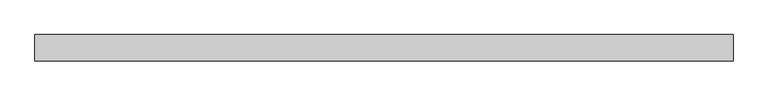
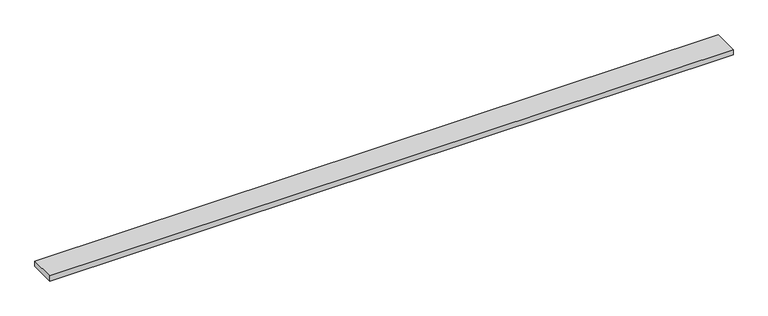
"""IFC4 building model written with IfcOpenShell, lengths in millimetres: proxy geometry, Generic Models 7:Generic Models 1:2:Generic Models 1:2 : Generic Models 7:Generic Models 1:337419:13 : Generic Models 7:Generic Models 1:2:Generic Models 1:2 : Generic Models 7:Generic Models 1:337419:306751."""

from ifc_helpers import new_model, si_unit, frame, origin, place, context, project, spatial, polyline, outline, extrude, source, transform, mapped, element, save


def generic_models_1bb8b360(model_context):
    return source(origin(), model_context, "Body", "SweptSolid", [
        extrude(outline(polyline([(596182.8367242, -536573.1495417), (596182.8367242, -536757.2995417), (591306.0367242, -536757.2995417), (591306.0367242, -536573.1495417), (596182.8367242, -536573.1495417)])), frame((0.0, 0.0, 2503.6859375), z_axis=(0.0, 0.0, 1.0), x_axis=(1.0, 0.0, 0.0)), (0.0, 0.0, 1.0), 38.1),
    ])


if __name__ == "__main__":
    model = new_model("IFC4")
    model_context = context("Model", 3, world=origin())
    ifc_project = project(units=[si_unit("LENGTHUNIT", "METRE", prefix="MILLI")], contexts=[model_context])
    site = spatial("IfcSite", under=ifc_project)
    building = spatial("IfcBuilding", under=site)
    placement = place(None, origin())
    generic_models_shape = generic_models_1bb8b360(model_context)
    element("IfcBuildingElementProxy", 1, Name="Generic Models 7:Generic Models 1:2:Generic Models 1:2 : Generic Models 7:Generic Models 1:337419:13 : Generic Models 7:Generic Models 1:2:Generic Models 1:2 : Generic Models 7:Generic Models 1:337419:306751", ObjectType="Generic Models 7:Generic Models 1:2:Generic Models 1:2 : Generic Models 7:Generic Models 1:337419:13 : Generic Models 7:Generic Models 1:2:Generic Models 1:2 : Generic Models 7:Generic Models 1:337419:306751", at=placement, inside=building, context=model_context, shape_type="MappedRepresentation", body=[
        mapped(generic_models_shape, transform((0.0, 0.0, 0.0), x_axis=(1.0, 0.0, 0.0), y_axis=(0.0, 1.0, 0.0), z_axis=(0.0, 0.0, 1.0))),
    ])
    save(model, "model.ifc")

# Revit data of these elements
# Type "Generic Models 7:Generic Models 1:2:Generic Models 1:2 : Generic Models 7:Generic Models 1:337419:13 : Generic Models 7:Generic Models 1:2:Generic Models 1:2 : Generic Models 7:Generic Models 1:337419:306751"
#   NameOverride = "Generic Models 7:Generic Models 1:2:Generic Models 1:2 : Generic Models 7:Generic Models 1:337419:306751"
#   ObjectTypeOverride = "Generic Models 1:2 : Generic Models 7:Generic Models 1:337419"
#   Reference = "Generic Models 1"
#   Tag = "306751"
# Element 1 (IfcBuildingElementProxy, "Generic Models 7:Generic Models 1:2:Generic Models 1:2 : Generic Models 7:Generic Models 1:337419:13 : Generic Models 7:Generic Models 1:2:Generic Models 1:2 : Generic Models 7:Generic Models 1:337419:306751")
#   Materials on its faces: "BLOCKING - SIZE AS NEC."
# Materials
#   "BLOCKING - SIZE AS NEC.": class "Wood", colour RGB 144 113 62, transparency 0, Description = "Pinus Echinata", Cost = 0
